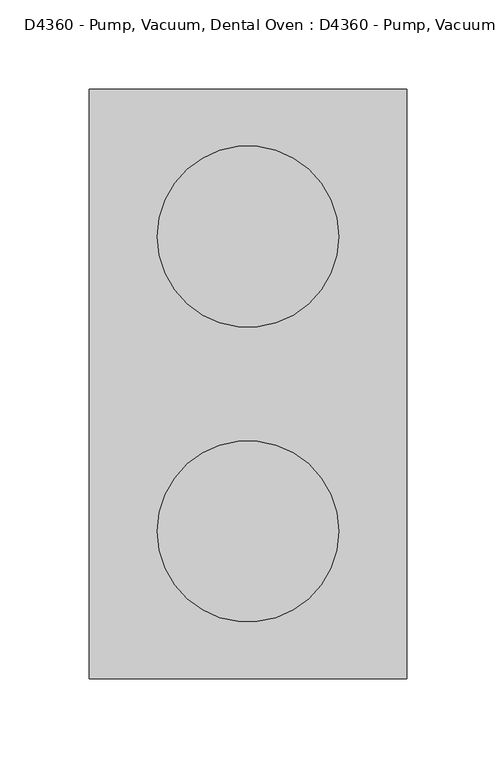
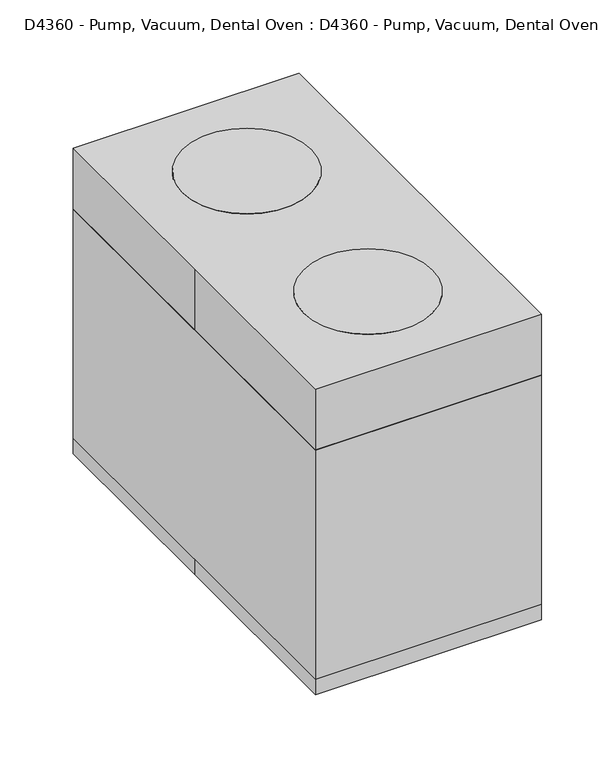
"""IFC4 building model written with IfcOpenShell, lengths in millimetres: proxy geometry, D4360 - Pump, Vacuum, Dental Oven : D4360 - Pump, Vacuum, Dental Oven."""

from ifc_helpers import new_model, si_unit, point, frame, frame_2d, origin, origin_with_axes, place, context, project, spatial, polyline, circle_curve, trimmed, segment, composite_curve, outline, extrude, source, transform, mapped, element, save


def d4360_pump_vacuum_dental_oven_d4360_pump_vacuum_dental_oven_7488b230(model_context):
    return source(origin(), model_context, "Body", "SweptSolid", [
        extrude(outline(composite_curve([segment(trimmed(circle_curve(frame_2d((0.0, -82.55)), 50.8), [point((-50.8, -82.55))], [point((50.8, -82.55))], False, "CARTESIAN"), True, "CONTINUOUS"), segment(trimmed(circle_curve(frame_2d((0.0, -82.55)), 50.8), [point((50.8, -82.55))], [point((-50.8, -82.55))], False, "CARTESIAN"), True, "CONTINUOUS")], self_intersect=False)), frame((0.0, 0.0, 203.2), z_axis=(0.0, 0.0, 1.0), x_axis=(1.0, 0.0, 0.0)), (0.0, 0.0, 1.0), 50.8),
        extrude(outline(polyline([(-70.7580755, 112.9852919), (-58.0580755, 112.9852919), (-58.0580755, -115.6147081), (-70.7580755, -115.6147081), (-70.7580755, 112.9852919)])), frame((0.0, 0.0, 203.2), z_axis=(0.0, 0.0, 1.0), x_axis=(1.0, 0.0, 0.0)), (0.0, 0.0, 1.0), 25.4),
        extrude(outline(polyline([(70.7580755, 112.9852919), (70.7580755, -115.6147081), (58.0580755, -115.6147081), (58.0580755, 112.9852919), (70.7580755, 112.9852919)])), frame((0.0, 0.0, 203.2), z_axis=(0.0, 0.0, 1.0), x_axis=(1.0, 0.0, 0.0)), (0.0, 0.0, 1.0), 25.4),
        extrude(outline(composite_curve([segment(trimmed(circle_curve(frame_2d((0.0, 82.55)), 50.8), [point((-50.8, 82.55))], [point((50.8, 82.55))], False, "CARTESIAN"), True, "CONTINUOUS"), segment(trimmed(circle_curve(frame_2d((0.0, 82.55)), 50.8), [point((50.8, 82.55))], [point((-50.8, 82.55))], False, "CARTESIAN"), True, "CONTINUOUS")], self_intersect=False)), frame((0.0, 0.0, 203.2), z_axis=(0.0, 0.0, 1.0), x_axis=(1.0, 0.0, 0.0)), (0.0, 0.0, 1.0), 50.8),
        extrude(outline(polyline([(88.9, 165.1), (88.9, -165.1), (-88.9, -165.1), (-88.9, 165.1), (88.9, 165.1)])), frame((0.0, 0.0, 12.7), z_axis=(0.0, 0.0, 1.0), x_axis=(1.0, 0.0, 0.0)), (0.0, 0.0, 1.0), 190.5),
        extrude(outline(composite_curve([segment(trimmed(circle_curve(frame_2d((-56.3344194, -133.8412182)), 12.7), [point((-43.6344194, -133.8412182))], [point((-69.0344194, -133.8412182))], False, "CARTESIAN"), True, "CONTINUOUS"), segment(trimmed(circle_curve(frame_2d((-56.3344194, -133.8412182)), 12.7), [point((-69.0344194, -133.8412182))], [point((-43.6344194, -133.8412182))], False, "CARTESIAN"), True, "CONTINUOUS")], self_intersect=False)), origin_with_axes(), (0.0, 0.0, 1.0), 12.7),
        extrude(outline(composite_curve([segment(trimmed(circle_curve(frame_2d((56.3344194, -133.8412182)), 12.7), [point((43.6344194, -133.8412182))], [point((69.0344194, -133.8412182))], False, "CARTESIAN"), True, "CONTINUOUS"), segment(trimmed(circle_curve(frame_2d((56.3344194, -133.8412182)), 12.7), [point((69.0344194, -133.8412182))], [point((43.6344194, -133.8412182))], False, "CARTESIAN"), True, "CONTINUOUS")], self_intersect=False)), origin_with_axes(), (0.0, 0.0, 1.0), 12.7),
        extrude(outline(composite_curve([segment(trimmed(circle_curve(frame_2d((-56.3344194, 133.8412182)), 12.7), [point((-43.6344194, 133.8412182))], [point((-69.0344194, 133.8412182))], False, "CARTESIAN"), True, "CONTINUOUS"), segment(trimmed(circle_curve(frame_2d((-56.3344194, 133.8412182)), 12.7), [point((-69.0344194, 133.8412182))], [point((-43.6344194, 133.8412182))], False, "CARTESIAN"), True, "CONTINUOUS")], self_intersect=False)), origin_with_axes(), (0.0, 0.0, 1.0), 12.7),
        extrude(outline(composite_curve([segment(trimmed(circle_curve(frame_2d((56.3344194, 133.8412182)), 12.7), [point((43.6344194, 133.8412182))], [point((69.0344194, 133.8412182))], False, "CARTESIAN"), True, "CONTINUOUS"), segment(trimmed(circle_curve(frame_2d((56.3344194, 133.8412182)), 12.7), [point((69.0344194, 133.8412182))], [point((43.6344194, 133.8412182))], False, "CARTESIAN"), True, "CONTINUOUS")], self_intersect=False)), origin_with_axes(), (0.0, 0.0, 1.0), 12.7),
        extrude(outline(polyline([(-88.9, 165.1), (88.9, 165.1), (88.9, -165.1), (-88.9, -165.1), (-88.9, 0.0), (-88.9, 165.1)])), origin_with_axes(), (0.0, 0.0, 1.0), 254.0),
    ])


if __name__ == "__main__":
    model = new_model("IFC4")
    model_context = context("Model", 3, world=origin())
    ifc_project = project(units=[si_unit("LENGTHUNIT", "METRE", prefix="MILLI")], contexts=[model_context])
    site = spatial("IfcSite", under=ifc_project)
    building = spatial("IfcBuilding", under=site)
    placement = place(None, origin())
    d4360_pump_vacuum_dental_oven_d4360_pump_vacuum_dental_oven_shape = d4360_pump_vacuum_dental_oven_d4360_pump_vacuum_dental_oven_7488b230(model_context)
    element("IfcBuildingElementProxy", 1, Name="D4360 - Pump, Vacuum, Dental Oven : D4360 - Pump, Vacuum, Dental Oven", ObjectType="D4360 - Pump, Vacuum, Dental Oven : D4360 - Pump, Vacuum, Dental Oven", at=placement, inside=building, context=model_context, shape_type="MappedRepresentation", body=[
        mapped(d4360_pump_vacuum_dental_oven_d4360_pump_vacuum_dental_oven_shape, transform((0.0, 0.0, 0.0), x_axis=(1.0, 0.0, 0.0), y_axis=(0.0, 1.0, 0.0), z_axis=(0.0, 0.0, 1.0))),
    ])
    save(model, "model.ifc")

# Revit data of these elements
# Type "D4360 - Pump, Vacuum, Dental Oven : D4360 - Pump, Vacuum, Dental Oven"
#   Watts2 = "0"
#   Watts1 = "480"
#   Unit_Issue = "EA"
#   UTIL_6_Misc = "-"
#   UTIL_5_NonMedGas = "-"
#   UTIL_4_MiscGas = "-"
#   UTIL_3_MedGas = "-"
#   UTIL_2_Elec = "A"
#   UTIL_1_WaterDrain = "-"
#   Nomenclature = "Pump, Vacuum, Dental Oven"
#   NSN = "6520"
#   Location [instance default] = ""
#   JSN = "D4360"
#   Fund_Source_VA = "-"
#   Fund_Source_Navy = "-"
#   Fund_Source_Army = "-"
#   Fund_Source_AF = "-"
#   ELEC_Volts2 = "0"
#   ELEC_Volts1 = "120"
#   ELEC_Phase2 = "0"
#   ELEC_Phase1 = "1"
#   ELEC_HertzSwitch = "0"
#   ELEC_HertzDependent = "-1"
#   ELEC_Hertz = "60"
#   ELEC_Amps2 = "0"
#   ELEC_Amps1 = "4"
#   DetailDescription = "Vacuum pump. The pump is used in dental laboratories to provide a vacuum source for the vacuum oven listed at JSN D4350."
#   CAT_VA = "C"
#   CAT_Navy = "C"
#   CAT_IHS = "-"
#   CAT_Army = "C"
#   CAT_AF = "C"
#   BTUperhour = "0"
#   Weight_IP = 21
#   DIM_Width_IP = 0' - 7"
#   DIM_Height_IP = 0' - 10"
#   DIM_Depth_IP = 1' - 1"
# Element 1 (IfcBuildingElementProxy, "D4360 - Pump, Vacuum, Dental Oven : D4360 - Pump, Vacuum, Dental Oven")
#   Location = "DNPC2"
#   Materials on its faces: "EquipSpace"
# Materials
#   "EquipSpace": class "Unassigned", colour RGB 221 217 195, transparency 0.5
